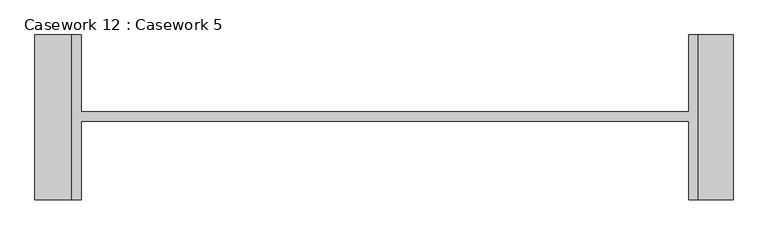
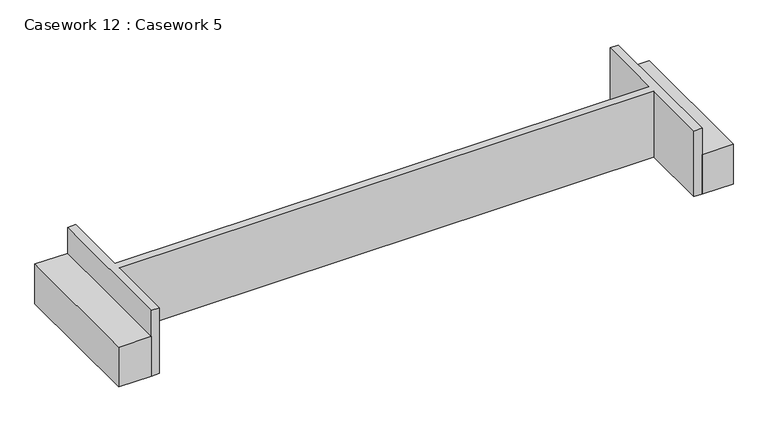
"""IFC4 building model written with IfcOpenShell, lengths in millimetres: furniture geometry, Casework 12 : Casework 5."""

from ifc_helpers import new_model, si_unit, origin, origin_with_axes, place, context, project, spatial, polyline, outline, extrude, source, transform, mapped, element, save


def casework_12_casework_5_6038fc15(model_context):
    return source(origin(), model_context, "Body", "SweptSolid", [
        extrude(outline(polyline([(-45222.23615, 264550.8000155), (-45222.23615, 262009.748706), (-45765.6431786, 262009.748706), (-45765.6431786, 264550.8000155), (-45222.23615, 264550.8000155)])), origin_with_axes(), (0.0, 0.0, 1.0), 736.6),
        extrude(outline(polyline([(-55407.3218514, 264550.8000155), (-55407.3218514, 262009.748706), (-55978.0010565, 262009.748706), (-55978.0010565, 264550.8000155), (-55407.3218514, 264550.8000155)])), origin_with_axes(), (0.0, 0.0, 1.0), 736.6),
        extrude(outline(polyline([(-55264.4443999, 264550.8000155), (-55264.4443999, 263363.5915012), (-45907.3606126, 263363.5915012), (-45907.3606126, 264550.8000155), (-45765.6431786, 264550.8000155), (-45765.6431786, 262009.748706), (-45907.3606126, 262009.748706), (-45907.3606126, 263221.7281826), (-55264.4443999, 263221.7281826), (-55264.4443999, 262009.748706), (-55407.3218514, 262009.748706), (-55407.3218514, 264550.8000155), (-55264.4443999, 264550.8000155)])), origin_with_axes(), (0.0, 0.0, 1.0), 1219.2),
    ])


if __name__ == "__main__":
    model = new_model("IFC4")
    model_context = context("Model", 3, world=origin())
    ifc_project = project(units=[si_unit("LENGTHUNIT", "METRE", prefix="MILLI")], contexts=[model_context])
    site = spatial("IfcSite", under=ifc_project)
    building = spatial("IfcBuilding", under=site)
    placement = place(None, origin())
    casework_12_casework_5_shape = casework_12_casework_5_6038fc15(model_context)
    element("IfcFurniture", 1, ObjectType="Casework 12 : Casework 5", at=placement, inside=building, context=model_context, shape_type="MappedRepresentation", body=[
        mapped(casework_12_casework_5_shape, transform((0.0, 0.0, 0.0), x_axis=(1.0, 0.0, 0.0), y_axis=(0.0, 1.0, 0.0), z_axis=(0.0, 0.0, 1.0))),
    ])
    save(model, "model.ifc")

# Revit data of these elements
# Element 1 (IfcFurniture, "Casework 12 : Casework 5")
#   Materials on its faces: "Casework-oakfire"
# Materials
#   "Casework-oakfire": class "Miscellaneous", colour RGB 164 164 164, transparency 0, Cost = 0
